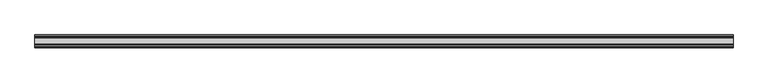
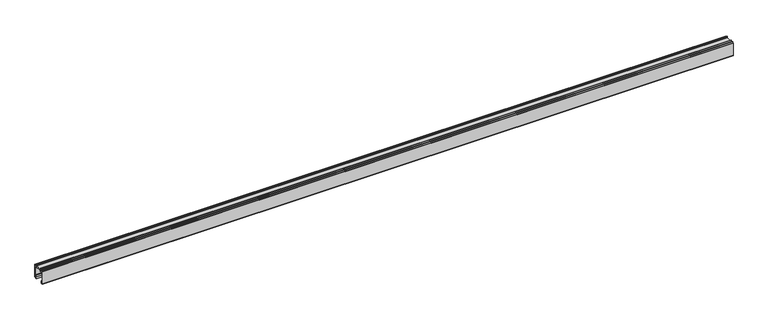
"""IFC4 building model written with IfcOpenShell, lengths in millimetres: proxy geometry, Generic Models 6:Generic Models 2:318829:Generic Models 2:318829 : Generic Models 6:Generic Models 2:318829:2 : Generic Models 6:Generic Models 2:318829:Generic Models 2:318829 : Generic Models 6:Generic Models 2:318829:300683."""

import ifcopenshell
import ifcopenshell.guid

model = None  # the IFC model being written
_history = None  # IfcOwnerHistory: only IFC2X3 demands one
_inside = {}  # id of a spatial element -> (the spatial element, [elements in it])
_under = {}  # id of a project, library or spatial element -> (it, [spatial elements below it])
_declared = {}  # id of a project -> (the project, [libraries it declares])
_typed = {}  # id of a type object -> (the type object, [elements of that type])
_made_of = {}  # id of a material, layer set ... -> (it, [elements and type objects made of it])


def new_model(schema):
    """Start an empty IFC model of exactly this schema.

    Asked for "IFC4X3", IfcOpenShell would pick the latest addendum, in which some entities
    have other attributes; the version numbers below select the first issue.
    IFC2X3 requires an IfcOwnerHistory on every rooted entity: one is made here for all.
    """
    global model, _history
    if schema == "IFC4X3":
        model = ifcopenshell.file(schema_version=(4, 3, 0, 0))
    else:
        model = ifcopenshell.file(schema=schema)
    _inside.clear()
    _under.clear()
    _declared.clear()
    _typed.clear()
    _made_of.clear()
    _history = None
    if model.schema == "IFC2X3":
        org = make("IfcOrganization", Name="unknown")
        user = make(
            "IfcPersonAndOrganization",
            ThePerson=make("IfcPerson", FamilyName="unknown"),
            TheOrganization=org,
        )
        app = make(
            "IfcApplication",
            ApplicationDeveloper=org,
            Version="unknown",
            ApplicationFullName="unknown",
            ApplicationIdentifier="unknown",
        )
        _history = make(
            "IfcOwnerHistory",
            OwningUser=user,
            OwningApplication=app,
            ChangeAction="ADDED",
            CreationDate=0,
        )
    return model


def make(cls, **values):
    """One entity of the class cls with the attributes given. An attribute that is None is left unset."""
    return model.create_entity(
        cls, **{name: value for name, value in values.items() if value is not None}
    )


def rooted(cls, **values):
    """An entity with a GlobalId (a new one), such as an element, a storey or a relation."""
    return make(cls, GlobalId=ifcopenshell.guid.new(), OwnerHistory=_history, **values)


def si_unit(unit_type, name, prefix=None):
    """IfcSIUnit, for example si_unit("LENGTHUNIT", "METRE", prefix="MILLI")."""
    return make("IfcSIUnit", UnitType=unit_type, Prefix=prefix, Name=name)


def assignment(units):
    """IfcUnitAssignment: the units of a project."""
    return None if units is None else make("IfcUnitAssignment", Units=units)


def point(xyz):
    """IfcCartesianPoint."""
    return None if xyz is None else make("IfcCartesianPoint", Coordinates=xyz)


def direction(xyz):
    """IfcDirection."""
    return None if xyz is None else make("IfcDirection", DirectionRatios=xyz)


def frame(location, z_axis=None, x_axis=None):
    """IfcAxis2Placement3D, a coordinate frame: its origin and axes. An axis left out is left unset."""
    return make(
        "IfcAxis2Placement3D",
        Location=point(location),
        Axis=direction(z_axis),
        RefDirection=direction(x_axis),
    )


def origin():
    """The frame at (0, 0, 0) with its axes left unset."""
    return frame((0.0, 0.0, 0.0))


def place(relative_to, where):
    """IfcLocalPlacement: puts the frame where relative to a parent placement (None: the world)."""
    return make(
        "IfcLocalPlacement", PlacementRelTo=relative_to, RelativePlacement=where
    )


def context(
    kind, dimensions, precision=None, world=None, true_north=None, identifier=None
):
    """IfcGeometricRepresentationContext, for example the 3D "Model" context."""
    return make(
        "IfcGeometricRepresentationContext",
        ContextIdentifier=identifier,
        ContextType=kind,
        CoordinateSpaceDimension=dimensions,
        Precision=precision,
        WorldCoordinateSystem=world,
        TrueNorth=true_north,
    )


def project(units=None, contexts=None):
    """IfcProject with its units and contexts."""
    return rooted(
        "IfcProject",
        Name="project",
        RepresentationContexts=contexts,
        UnitsInContext=assignment(units),
    )


def spatial(cls, under=None, at=None, **own):
    """A site, building, storey or space (cls), placed at a placement, below another one or the project."""
    s = rooted(cls, ObjectPlacement=at, **own)
    if under is not None:
        _under.setdefault(under.id(), (under, []))[1].append(s)
    return s


def polyline(points):
    """IfcPolyline through the points."""
    return make("IfcPolyline", Points=[point(p) for p in points])


def outline(outer, holes=None, kind="AREA"):
    """IfcArbitraryClosedProfileDef: a profile drawn as a closed curve; with holes, ...WithVoids."""
    if holes is None:
        return make("IfcArbitraryClosedProfileDef", ProfileType=kind, OuterCurve=outer)
    return make(
        "IfcArbitraryProfileDefWithVoids",
        ProfileType=kind,
        OuterCurve=outer,
        InnerCurves=holes,
    )


def extrude(swept, where, along, depth):
    """IfcExtrudedAreaSolid: the profile swept, set in the frame where, extruded along a direction by depth."""
    return make(
        "IfcExtrudedAreaSolid",
        SweptArea=swept,
        Position=where,
        ExtrudedDirection=direction(along),
        Depth=depth,
    )


def shape(context_of_items, identifier, shape_type, items):
    """IfcShapeRepresentation: the items that make up one representation, for example the "Body"."""
    return make(
        "IfcShapeRepresentation",
        ContextOfItems=context_of_items,
        RepresentationIdentifier=identifier,
        RepresentationType=shape_type,
        Items=items,
    )


def source(mapping_origin, context_of_items, identifier, shape_type, items):
    """IfcRepresentationMap: a shape defined once, which mapped items show again and again."""
    return make(
        "IfcRepresentationMap",
        MappingOrigin=mapping_origin,
        MappedRepresentation=shape(context_of_items, identifier, shape_type, items),
    )


def transform(
    local_origin,
    x_axis=None,
    y_axis=None,
    z_axis=None,
    scale=None,
    scale2=None,
    scale3=None,
    uniform=True,
):
    """IfcCartesianTransformationOperator3D, or its non-uniform kind. x_axis, y_axis, z_axis: its Axis1, 2, 3."""
    if uniform:
        return make(
            "IfcCartesianTransformationOperator3D",
            Axis1=direction(x_axis),
            Axis2=direction(y_axis),
            LocalOrigin=point(local_origin),
            Scale=scale,
            Axis3=direction(z_axis),
        )
    return make(
        "IfcCartesianTransformationOperator3DnonUniform",
        Axis1=direction(x_axis),
        Axis2=direction(y_axis),
        LocalOrigin=point(local_origin),
        Scale=scale,
        Axis3=direction(z_axis),
        Scale2=scale2,
        Scale3=scale3,
    )


def mapped(mapping_source, mapping_target):
    """IfcMappedItem: shows the shape of a source again, moved by a transform."""
    return make(
        "IfcMappedItem", MappingSource=mapping_source, MappingTarget=mapping_target
    )


def made_of(thing, what):
    """Note that an element or type object is made of a material, layer set ...; save() writes the relation."""
    if what is not None:
        _made_of.setdefault(what.id(), (what, []))[1].append(thing)
    return thing


def element(
    cls,
    number,
    at=None,
    inside=None,
    cuts=None,
    type_object=None,
    material=None,
    context=None,
    identifier="Body",
    shape_type=None,
    held_by="IfcProductDefinitionShape",
    body=None,
    shapes=None,
    **own,
):
    """One element of the class cls, such as IfcWall. Its Tag is "e" and its number.

    at: its placement. inside: the storey or other place that contains it. cuts: it is an
    opening in that element (IfcRelVoidsElement). A single representation is given by context,
    identifier, shape_type and body (its items); several are given by shapes. held_by: the class
    of the entity that holds the representations. save() writes the other relations.
    """
    e = rooted(cls, Tag="e%d" % number, ObjectPlacement=at, **own)
    if body is not None:
        shapes = [shape(context, identifier, shape_type, body)]
    if shapes is not None:
        e.Representation = make(held_by, Representations=shapes)
    if inside is not None:
        _inside.setdefault(inside.id(), (inside, []))[1].append(e)
    if cuts is not None:
        rooted(
            "IfcRelVoidsElement", RelatingBuildingElement=cuts, RelatedOpeningElement=e
        )
    if type_object is not None:
        _typed.setdefault(type_object.id(), (type_object, []))[1].append(e)
    return made_of(e, material)


def aggregate(whole, parts):
    """IfcRelAggregates: a whole, such as a stair, and the parts it consists of."""
    return rooted("IfcRelAggregates", RelatingObject=whole, RelatedObjects=parts)


def save(model, path):
    """Write the relations noted so far, then the file.

    IfcRelAggregates (storeys below a building ...), IfcRelContainedInSpatialStructure (elements
    in a storey), IfcRelDefinesByType, IfcRelAssociatesMaterial and IfcRelDeclares: one each for
    every whole, place, type object, material and project.
    """
    for whole, parts in _under.values():
        aggregate(whole, parts)
    for where, things in _inside.values():
        rooted(
            "IfcRelContainedInSpatialStructure",
            RelatedElements=things,
            RelatingStructure=where,
        )
    for kind, things in _typed.values():
        rooted("IfcRelDefinesByType", RelatedObjects=things, RelatingType=kind)
    for what, things in _made_of.values():
        rooted("IfcRelAssociatesMaterial", RelatedObjects=things, RelatingMaterial=what)
    for by, libraries in _declared.values():
        rooted("IfcRelDeclares", RelatingContext=by, RelatedDefinitions=libraries)
    model.write(path)


def generic_models_c3fbaf1e(model_context):
    return source(origin(), model_context, "Body", "SweptSolid", [
        extrude(outline(polyline([(-536498.4587882, 10076.5121428), (-536498.5080328, 10077.4620117), (-536497.7674778, 10077.955715), (-536496.7541511, 10077.2970526), (-536495.3462744, 10077.2970526), (-536495.3462744, 10079.6093776), (-536492.2038841, 10079.6093776), (-536492.2038841, 10015.101441), (-536497.6585993, 10015.101441), (-536497.6585993, 10018.2438313), (-536495.8798878, 10018.5402832), (-536497.6585993, 10023.4020946), (-536497.6585993, 10027.6710022), (-536495.3462744, 10027.6710022), (-536495.3462744, 10072.1980797), (-536507.5008029, 10072.1980797), (-536507.5008029, 10073.5702286), (-536497.5993089, 10074.9847277), (-536497.5993089, 10076.0355147), (-536498.4587882, 10076.5121428)])), frame((592370.1456333, 0.0, 0.0), z_axis=(1.0, 0.0, 0.0), x_axis=(0.0, 1.0, 0.0)), (0.0, 0.0, 1.0), 3417.2905312),
        extrude(outline(polyline([(-536493.8163228, 10013.8651082), (-536505.2477683, 10010.8167227), (-536505.2477683, 10022.4223357), (-536499.1544889, 10027.6710022), (-536497.9491849, 10027.6710022), (-536497.9491849, 10023.141866), (-536496.407148, 10018.9269652), (-536497.9491849, 10018.6699591), (-536497.9491849, 10014.9037213), (-536493.8163228, 10014.9037213), (-536493.8163228, 10013.8651082)])), frame((592370.1456333, 0.0, 0.0), z_axis=(1.0, 0.0, 0.0), x_axis=(0.0, 1.0, 0.0)), (0.0, 0.0, 1.0), 3417.2905312),
        extrude(outline(polyline([(-536553.1543976, 10026.9595176), (-536548.5890382, 10026.9595176), (-536548.5890382, 10024.913923), (-536549.8934266, 10023.6096505), (-536549.8934266, 10025.4179677), (-536551.3756861, 10025.4179677), (-536552.3695065, 10023.6966203), (-536552.3695065, 10021.4152012), (-536551.4840848, 10019.5164082), (-536549.8934266, 10019.5164082), (-536549.8934266, 10021.5496317), (-536548.5890382, 10021.3269312), (-536548.5890382, 10016.2872487), (-536555.7038841, 10016.8856937), (-536555.7038841, 10079.3129256), (-536552.1464611, 10079.3129256), (-536552.1464611, 10085.5977062), (-536550.1305881, 10085.5977062), (-536550.1305881, 10079.3129256), (-536539.2211577, 10079.3129256), (-536539.2211577, 10085.5977062), (-536537.2052846, 10085.5977062), (-536537.2052846, 10079.3129256), (-536506.1371241, 10079.3129256), (-536506.1371241, 10085.5977062), (-536504.121251, 10085.5977062), (-536504.121251, 10079.3129256), (-536495.5241455, 10079.3129256), (-536495.5241455, 10077.9492468), (-536496.3542109, 10077.4156334), (-536497.302857, 10078.0678276), (-536504.121251, 10078.0678276), (-536505.4256395, 10076.7634392), (-536509.1609336, 10076.7634392), (-536509.1609336, 10071.4273047), (-536495.7020167, 10071.4273047), (-536495.7020167, 10069.8857548), (-536511.1768066, 10069.8857548), (-536511.1768066, 10076.7634392), (-536537.0867039, 10076.7634392), (-536537.0867039, 10069.8857548), (-536553.1543976, 10069.8857548), (-536553.1543976, 10026.9595176)]), holes=[polyline([(-536552.5614938, 10077.1784719), (-536552.5614938, 10071.4273047), (-536539.2211577, 10071.4273047), (-536539.2211577, 10077.1784719), (-536552.5614938, 10077.1784719)])]), frame((592370.1456333, 0.0, 0.0), z_axis=(1.0, 0.0, 0.0), x_axis=(0.0, 1.0, 0.0)), (0.0, 0.0, 1.0), 3417.2905312),
        extrude(outline(polyline([(-536545.2477683, 10012.3068987), (-536555.2064077, 10014.525663), (-536555.2064077, 10016.6270779), (-536548.2821927, 10016.0446673), (-536548.2821927, 10021.4849671), (-536550.2058448, 10021.8133955), (-536550.2058448, 10019.7751321), (-536551.2301937, 10019.7751321), (-536552.0702393, 10021.5766157), (-536552.0702393, 10023.6569142), (-536551.209791, 10025.1472545), (-536550.1206041, 10025.1472545), (-536550.1206041, 10022.8928663), (-536548.2821927, 10024.7312777), (-536548.2821927, 10026.9595176), (-536545.2477683, 10026.9595176), (-536545.2477683, 10012.3068987)])), frame((592370.1456333, 0.0, 0.0), z_axis=(1.0, 0.0, 0.0), x_axis=(0.0, 1.0, 0.0)), (0.0, 0.0, 1.0), 3417.2905312),
    ])


if __name__ == "__main__":
    model = new_model("IFC4")
    model_context = context("Model", 3, world=origin())
    ifc_project = project(units=[si_unit("LENGTHUNIT", "METRE", prefix="MILLI")], contexts=[model_context])
    site = spatial("IfcSite", under=ifc_project)
    building = spatial("IfcBuilding", under=site)
    placement = place(None, origin())
    generic_models_shape = generic_models_c3fbaf1e(model_context)
    element("IfcBuildingElementProxy", 1, Name="Generic Models 6:Generic Models 2:318829:Generic Models 2:318829 : Generic Models 6:Generic Models 2:318829:2 : Generic Models 6:Generic Models 2:318829:Generic Models 2:318829 : Generic Models 6:Generic Models 2:318829:300683", ObjectType="Generic Models 6:Generic Models 2:318829:Generic Models 2:318829 : Generic Models 6:Generic Models 2:318829:2 : Generic Models 6:Generic Models 2:318829:Generic Models 2:318829 : Generic Models 6:Generic Models 2:318829:300683", at=placement, inside=building, context=model_context, shape_type="MappedRepresentation", body=[
        mapped(generic_models_shape, transform((0.0, 0.0, 0.0), x_axis=(1.0, 0.0, 0.0), y_axis=(0.0, 1.0, 0.0), z_axis=(0.0, 0.0, 1.0))),
    ])
    save(model, "model.ifc")

# Revit data of these elements
# Type "Generic Models 6:Generic Models 2:318829:Generic Models 2:318829 : Generic Models 6:Generic Models 2:318829:2 : Generic Models 6:Generic Models 2:318829:Generic Models 2:318829 : Generic Models 6:Generic Models 2:318829:300683"
#   NameOverride = "Generic Models 6:Generic Models 2:318829:Generic Models 2:318829 : Generic Models 6:Generic Models 2:318829:300683"
#   ObjectTypeOverride = "Generic Models 2:318829 : Generic Models 6:Generic Models 2:318829"
#   Reference = "Generic Models 2"
#   Tag = "300683"
# Element 1 (IfcBuildingElementProxy, "Generic Models 6:Generic Models 2:318829:Generic Models 2:318829 : Generic Models 6:Generic Models 2:318829:2 : Generic Models 6:Generic Models 2:318829:Generic Models 2:318829 : Generic Models 6:Generic Models 2:318829:300683")
#   Materials on its faces: "THERMAL BROKEN ALUMINUM STOREFRONT FOR POLYCARBONATE"
# Materials
#   "THERMAL BROKEN ALUMINUM STOREFRONT FOR POLYCARBONATE": class "Unassigned", colour RGB 244 244 244, transparency 0, Keynote = "M07611300.01", Cost = 0
